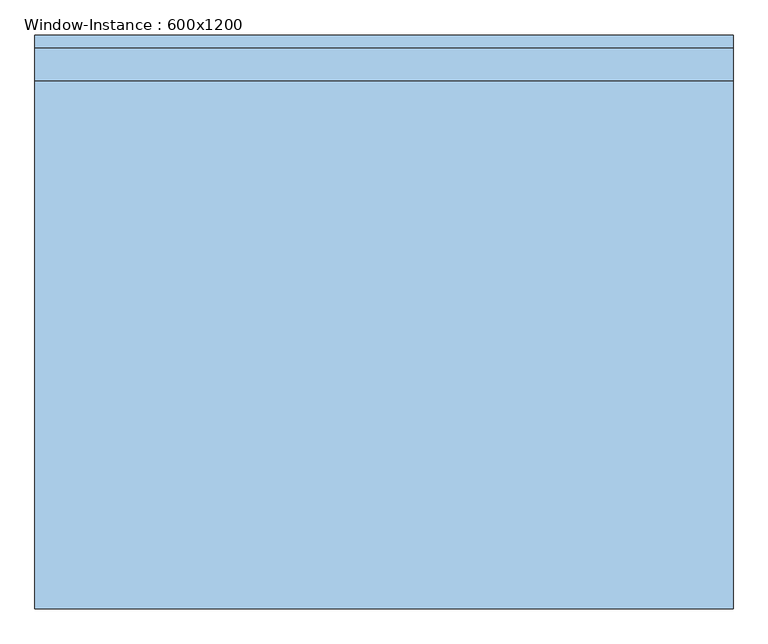
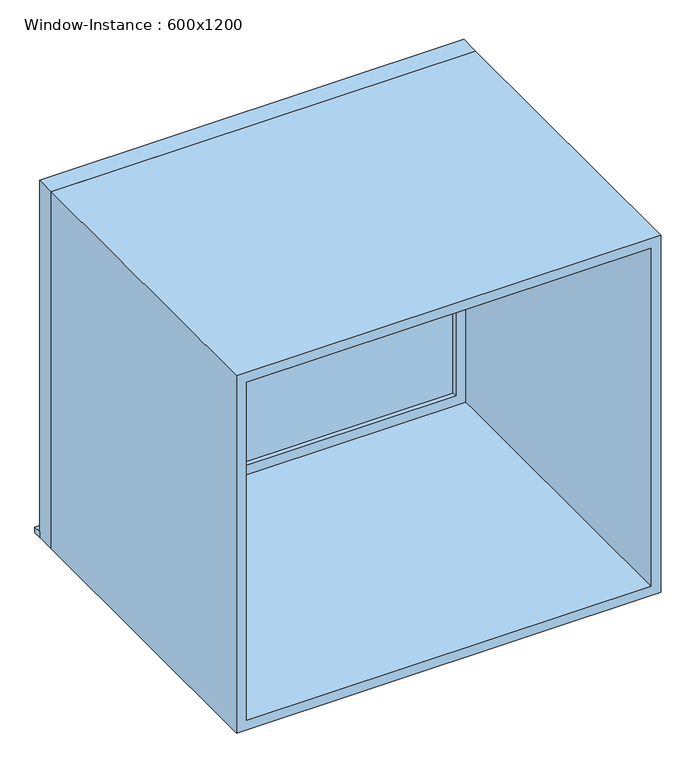
"""IFC4 building model written with IfcOpenShell, lengths in millimetres: window geometry, Window-Instance : 600x1200."""

from ifc_helpers import new_model, si_unit, frame, origin, place, context, project, spatial, polyline, outline, extrude, source, transform, mapped, element, save


def window_instance_600x1200_86a208f5(model_context):
    return source(origin(), model_context, "Body", "SweptSolid", [
        extrude(outline(polyline([(-713.1, 567.9), (636.9, 567.9), (636.9, 542.5), (-713.1, 542.5), (-713.1, 567.9)])), frame((0.0, 0.0, 900.0), z_axis=(0.0, 0.0, 1.0), x_axis=(1.0, 0.0, 0.0)), (0.0, 0.0, 1.0), 19.05),
        extrude(outline(polyline([(573.4, 493.925), (-649.6, 493.925), (-649.6, 506.625), (573.4, 506.625), (573.4, 493.925)])), frame((0.0, 0.0, 963.5), z_axis=(0.0, 0.0, 1.0), x_axis=(1.0, 0.0, 0.0)), (0.0, 0.0, 1.0), 1073.0),
        extrude(outline(polyline([(2080.95, -694.05), (919.05, -694.05), (919.05, 617.85), (2080.95, 617.85), (2080.95, -694.05)]), holes=[polyline([(2036.5, -649.6), (2036.5, 573.4), (963.5, 573.4), (963.5, -649.6), (2036.5, -649.6)])]), frame((0.0, 478.05, 0.0), z_axis=(0.0, 1.0, 0.0), x_axis=(0.0, 0.0, 1.0)), (0.0, 0.0, 1.0), 44.45),
        extrude(outline(polyline([(2100.0, -713.1), (900.0, -713.1), (900.0, 636.9), (2100.0, 636.9), (2100.0, -713.1)]), holes=[polyline([(2068.25, -681.35), (2068.25, 605.15), (931.75, 605.15), (931.75, -681.35), (2068.25, -681.35)])]), frame((0.0, -542.5, 0.0), z_axis=(0.0, 1.0, 0.0), x_axis=(0.0, 0.0, 1.0)), (0.0, 0.0, 1.0), 1020.55),
        extrude(outline(polyline([(2100.0, 636.9), (2100.0, -713.1), (900.0, -713.1), (900.0, 636.9), (2100.0, 636.9)]), holes=[polyline([(2080.95, 617.85), (919.05, 617.85), (919.05, -694.05), (2080.95, -694.05), (2080.95, 617.85)])]), frame((0.0, 478.05, 0.0), z_axis=(0.0, 1.0, 0.0), x_axis=(0.0, 0.0, 1.0)), (0.0, 0.0, 1.0), 64.45),
    ])


if __name__ == "__main__":
    model = new_model("IFC4")
    model_context = context("Model", 3, world=origin())
    ifc_project = project(units=[si_unit("LENGTHUNIT", "METRE", prefix="MILLI")], contexts=[model_context])
    site = spatial("IfcSite", under=ifc_project)
    building = spatial("IfcBuilding", under=site)
    placement = place(None, origin())
    window_instance_600x1200_shape = window_instance_600x1200_86a208f5(model_context)
    element("IfcWindow", 1, ObjectType="Window-Instance : 600x1200", at=placement, inside=building, context=model_context, shape_type="MappedRepresentation", body=[
        mapped(window_instance_600x1200_shape, transform((0.0, 0.0, 0.0), x_axis=(1.0, 0.0, 0.0), y_axis=(0.0, 1.0, 0.0), z_axis=(0.0, 0.0, 1.0))),
    ])
    save(model, "model.ifc")

# Revit data of these elements
# Type "Window-Instance : 600x1200"
#   Type Mark = "7"
#   Construction Type Id = "GSP4R"
#   Assembly Code = "B2020100"
#   Analytic Construction = "1/8 in Pilkington single glazing"
#   Visual Light Transmittance = 0.9
#   Thermal Resistance (R) = 0.149095 (m²·K)/W
#   Solar Heat Gain Coefficient = 0.86
#   Heat Transfer Coefficient (U) = 6.70716 W/(m²·K)
#   Height [instance default] = 1200 mm
#   Default Sill Height = 900 mm
#   Width [instance default] = 600 mm
#   Window Inset = 20 mm
#   Glass Pane Material = WW-EC-GL-Storefront
#   Sash Material = WW-EC-RGB-White
#   Wall Closure = (empty or 0)
# Element 1 (IfcWindow, "Window-Instance : 600x1200")
#   Width = 1350 mm
#   Materials on its faces: "WW-EC-RGB-White", "WW-EC-GL-Storefront"
# Materials
#   "WW-EC-GL-Storefront": class "Glass", colour RGB 236 240 239, transparency 0.85, Description = "Storefront Glass", Cost = 0
#   "WW-EC-RGB-White": class "Generic", colour RGB 255 255 255, transparency 0, Comments = "If region requests off-white, swith asset color to RGB 231-228-220", Description = "Generic Color", Cost = 0
